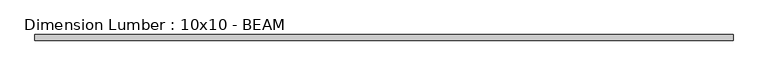
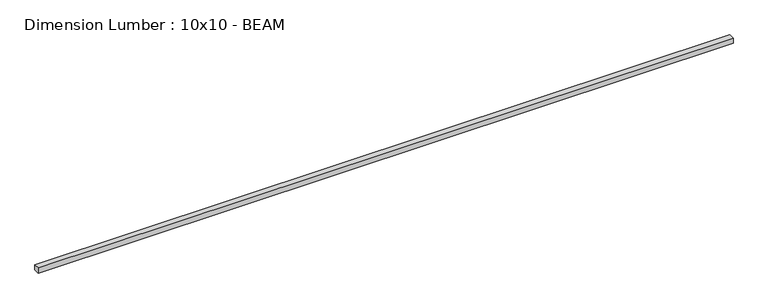
"""IFC4 building model written with IfcOpenShell, lengths in millimetres: beam geometry, Dimension Lumber : 10x10 - BEAM."""

from ifc_helpers import new_model, si_unit, frame, origin, place, context, project, spatial, polyline, outline, extrude, source, transform, mapped, element, save


def dimension_lumber_10x10_beam_bd205abd(model_context):
    return source(origin(), model_context, "Body", "SweptSolid", [
        extrude(outline(polyline([(14564.075555, 117.475), (14564.075555, -117.475), (-14467.238055, -117.475), (-14467.238055, 117.475), (14564.075555, 117.475)])), frame((0.0, 0.0, -117.475), z_axis=(0.0, 0.0, 1.0), x_axis=(1.0, 0.0, 0.0)), (0.0, 0.0, 1.0), 234.95),
    ])


if __name__ == "__main__":
    model = new_model("IFC4")
    model_context = context("Model", 3, world=origin())
    ifc_project = project(units=[si_unit("LENGTHUNIT", "METRE", prefix="MILLI")], contexts=[model_context])
    site = spatial("IfcSite", under=ifc_project)
    building = spatial("IfcBuilding", under=site)
    placement = place(None, origin())
    dimension_lumber_10x10_beam_shape = dimension_lumber_10x10_beam_bd205abd(model_context)
    element("IfcBeam", 1, ObjectType="Dimension Lumber : 10x10 - BEAM", at=placement, inside=building, context=model_context, shape_type="MappedRepresentation", body=[
        mapped(dimension_lumber_10x10_beam_shape, transform((0.0, 0.0, 0.0), x_axis=(1.0, 0.0, 0.0), y_axis=(0.0, 1.0, 0.0), z_axis=(0.0, 0.0, 1.0))),
    ])
    save(model, "model.ifc")

# Revit data of these elements
# Type "Dimension Lumber : 10x10 - BEAM"
#   Assembly Code = "B10"
#   A = 0.0755556 SF
#   Length [instance default] = 5' - 0"
#   b = 0' - 9 1/4"
#   d = 0' - 9 1/4"
#   Structural Material = (4) CHARRED SISTERED 2X10s AT BEAM
# Element 1 (IfcBeam, "Dimension Lumber : 10x10 - BEAM")
#   Materials on its faces: "(4) CHARRED SISTERED 2X10s AT BEAM"
# Materials
#   "(4) CHARRED SISTERED 2X10s AT BEAM": class "Wood", colour RGB 144 144 144, transparency 0, Description = "Pinus Echinata", Cost = 0
